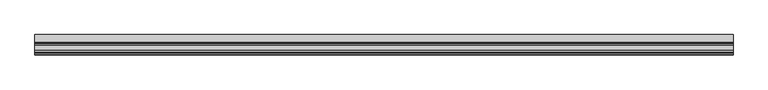
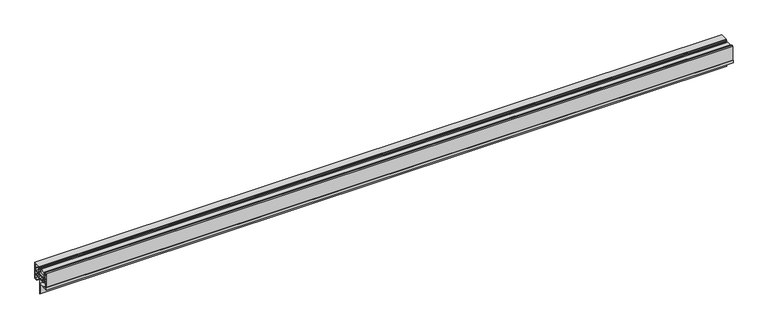
"""IFC4 building model written with IfcOpenShell, lengths in millimetres: proxy geometry, Window frame004 1637 : Window frame004 1637."""

from ifc_helpers import new_model, si_unit, frame, origin, place, context, project, spatial, polyline, outline, extrude, source, transform, mapped, element, save


def generic_models_991ec7d0(model_context):
    return source(origin(), model_context, "Body", "SweptSolid", [
        extrude(outline(polyline([(9723.7713026, 37545.1566334), (9723.7713026, 37547.5696334), (9725.9975166, 37547.5696334), (9726.4212579, 37550.0285263), (9727.7746229, 37550.0285263), (9728.4102621, 37547.1665501), (9728.4102621, 37545.3051872), (9727.747735, 37542.7149696), (9726.5736227, 37542.7149696), (9725.9982105, 37545.1566334), (9723.7713026, 37545.1566334)])), frame((3694.2883192, 0.0, 0.0), z_axis=(1.0, 0.0, 0.0), x_axis=(0.0, 1.0, 0.0)), (0.0, 0.0, 1.0), 2000.0),
        extrude(outline(polyline([(9758.5185026, 37547.5868625), (9758.5185026, 37545.1738625), (9756.2922886, 37545.1738625), (9755.8685473, 37542.7149696), (9754.5151824, 37542.7149696), (9753.8795432, 37545.5769458), (9753.8795432, 37547.4383087), (9754.5420703, 37550.0285263), (9755.7161826, 37550.0285263), (9756.2915948, 37547.5868625), (9758.5185026, 37547.5868625)])), frame((3694.2883192, 0.0, 0.0), z_axis=(1.0, 0.0, 0.0), x_axis=(0.0, 1.0, 0.0)), (0.0, 0.0, 1.0), 2000.0),
        extrude(outline(polyline([(3694.2883192, 9734.7568026), (3694.2883192, 9747.5330026), (5694.2883192, 9747.5330026), (5694.2883192, 9734.7568026), (3694.2883192, 9734.7568026)])), frame((0.0, 0.0, 37537.4903625), z_axis=(0.0, 0.0, 1.0), x_axis=(1.0, 0.0, 0.0)), (0.0, 0.0, 1.0), 9.525),
        extrude(outline(polyline([(9739.8141425, 37529.7433625), (9739.8141425, 37531.6119447), (9732.9007638, 37531.6119447), (9732.9007638, 37527.9145625), (9726.0827026, 37527.9145625), (9726.0827026, 37531.1931991), (9727.984619, 37531.1931991), (9727.984619, 37535.964471), (9729.749919, 37537.4903625), (9753.8576026, 37537.4903625), (9753.8576026, 37529.7433625), (9739.8141425, 37529.7433625)])), frame((3694.2883192, 0.0, 0.0), z_axis=(1.0, 0.0, 0.0), x_axis=(0.0, 1.0, 0.0)), (0.0, 0.0, 1.0), 2000.0),
        extrude(outline(polyline([(9775.4735631, 37532.7405625), (9776.4005173, 37530.6829834), (9775.3390149, 37529.0664558), (9774.0508822, 37529.0664558), (9774.0508822, 37534.1375625), (9777.4415026, 37534.1375625), (9777.4415026, 37548.7933625), (9760.1695026, 37548.7933625), (9760.1695026, 37528.3463625), (9736.1518446, 37528.3463625), (9736.1518446, 37529.7179625), (9758.7725026, 37529.7179625), (9758.7725026, 37542.5703625), (9756.2325026, 37542.5703625), (9756.2325026, 37544.7466583), (9757.5008807, 37544.7466583), (9757.5008807, 37543.8403625), (9758.7725026, 37543.8403625), (9758.7725026, 37548.9203625), (9757.5008807, 37548.9203625), (9757.5008807, 37547.9988632), (9756.2325026, 37547.9988632), (9756.2325026, 37550.1903625), (9778.8385026, 37550.1903625), (9778.8385026, 37532.7405625), (9775.4735631, 37532.7405625)])), frame((3694.2883192, 0.0, 0.0), z_axis=(1.0, 0.0, 0.0), x_axis=(0.0, 1.0, 0.0)), (0.0, 0.0, 1.0), 2000.0),
        extrude(outline(polyline([(9737.6905026, 37516.3321625), (9737.6905026, 37525.8825625), (9733.1012905, 37525.8825625), (9733.1012905, 37527.9145625), (9734.6416892, 37527.9145625), (9734.6416892, 37531.0895625), (9739.0893772, 37531.0895625), (9739.0893772, 37529.7433625), (9736.1518446, 37529.7433625), (9736.1518446, 37527.9145625), (9776.8065026, 37527.9145625), (9776.8065026, 37530.1748048), (9775.551216, 37532.7405625), (9778.8385026, 37532.7405625), (9778.8385026, 37501.1175625), (9768.3483026, 37501.1175625), (9768.3483026, 37503.1495625), (9776.8065026, 37503.1495625), (9776.5525026, 37514.3001625), (9755.0133026, 37514.3001625), (9755.0133026, 37470.7700298), (9753.4385031, 37470.7700298), (9753.4385031, 37514.3001625), (9733.8805026, 37514.3001625), (9733.8805026, 37517.8693733), (9735.1468473, 37517.8693733), (9735.1468473, 37516.3321625), (9737.6905026, 37516.3321625)]), holes=[polyline([(9772.8162468, 37516.3321625), (9776.2985026, 37516.3321625), (9776.2985026, 37525.8825625), (9772.8162468, 37525.8825625), (9772.8162468, 37524.7395625), (9762.8774031, 37524.7395625), (9762.8774031, 37525.8825625), (9759.2470473, 37525.8825625), (9759.2470473, 37524.7395625), (9754.0989026, 37524.7395625), (9754.0989026, 37525.8825625), (9747.2851294, 37525.8825625), (9747.2851294, 37524.7395625), (9739.7225026, 37524.7395625), (9739.7225026, 37517.4751625), (9743.6845244, 37517.4751625), (9743.6845244, 37516.3321625), (9752.6705617, 37516.3321625), (9752.6705617, 37517.4751625), (9759.2470473, 37517.4751625), (9759.2470473, 37516.3321625), (9767.4897498, 37516.3321625), (9767.4897498, 37517.4751625), (9772.8162468, 37517.4751625), (9772.8162468, 37516.3321625)])]), frame((3694.2883192, 0.0, 0.0), z_axis=(1.0, 0.0, 0.0), x_axis=(0.0, 1.0, 0.0)), (0.0, 0.0, 1.0), 2000.0),
        extrude(outline(polyline([(9721.6885026, 37501.1175625), (9753.4385026, 37501.1175625), (9753.4385026, 37469.3675625), (9752.4225026, 37469.3675625), (9752.4225026, 37500.1015625), (9720.6725026, 37500.1015625), (9720.6725026, 37507.4675625), (9721.6885026, 37507.4675625), (9721.6885026, 37501.1175625)])), frame((3694.2883192, 0.0, 0.0), z_axis=(1.0, 0.0, 0.0), x_axis=(0.0, 1.0, 0.0)), (0.0, 0.0, 1.0), 2000.0),
        extrude(outline(polyline([(9721.6885026, 37550.1903625), (9726.0827026, 37550.1903625), (9726.0827026, 37548.0609092), (9724.8127026, 37548.0609092), (9724.8127026, 37548.9203625), (9723.5427026, 37548.9203625), (9723.5427026, 37543.8403625), (9724.8127026, 37543.8403625), (9724.8127026, 37544.6984291), (9726.0827026, 37544.6984291), (9726.0827026, 37527.9145625), (9728.3097148, 37527.9145625), (9728.3097148, 37525.8825625), (9723.7205026, 37525.8825625), (9723.7205026, 37516.3321625), (9726.186283, 37516.3321625), (9726.186283, 37517.8693733), (9727.5305026, 37517.8693733), (9727.5305026, 37514.3001625), (9723.7205026, 37514.3001625), (9723.7205026, 37503.1495625), (9731.9247026, 37503.1495625), (9731.9247026, 37501.1175625), (9721.6885026, 37501.1175625), (9721.6885026, 37550.1903625)])), frame((3694.2883192, 0.0, 0.0), z_axis=(1.0, 0.0, 0.0), x_axis=(0.0, 1.0, 0.0)), (0.0, 0.0, 1.0), 2000.0),
    ])


if __name__ == "__main__":
    model = new_model("IFC4")
    model_context = context("Model", 3, world=origin())
    ifc_project = project(units=[si_unit("LENGTHUNIT", "METRE", prefix="MILLI")], contexts=[model_context])
    site = spatial("IfcSite", under=ifc_project)
    building = spatial("IfcBuilding", under=site)
    placement = place(None, origin())
    generic_models_shape = generic_models_991ec7d0(model_context)
    element("IfcBuildingElementProxy", 1, Name="Window frame004 1637 : Window frame004 1637", ObjectType="Window frame004 1637 : Window frame004 1637", at=placement, inside=building, context=model_context, shape_type="MappedRepresentation", body=[
        mapped(generic_models_shape, transform((0.0, 0.0, 0.0), x_axis=(1.0, 0.0, 0.0), y_axis=(0.0, 1.0, 0.0), z_axis=(0.0, 0.0, 1.0))),
    ])
    save(model, "model.ifc")

# Revit data of these elements
# Type "Window frame004 1637 : Window frame004 1637"
#   NameOverride = "Window frame004"
# Element 1 (IfcBuildingElementProxy, "Window frame004 1637 : Window frame004 1637")
#   Materials on its faces: "FLEETWOOD SERIES 250-T-04 FIXED UNIT WINDOW FRAME"
# Materials
#   "FLEETWOOD SERIES 250-T-04 FIXED UNIT WINDOW FRAME": class "Unassigned", colour RGB 128 128 128, transparency 0
